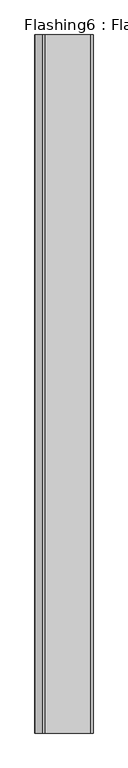
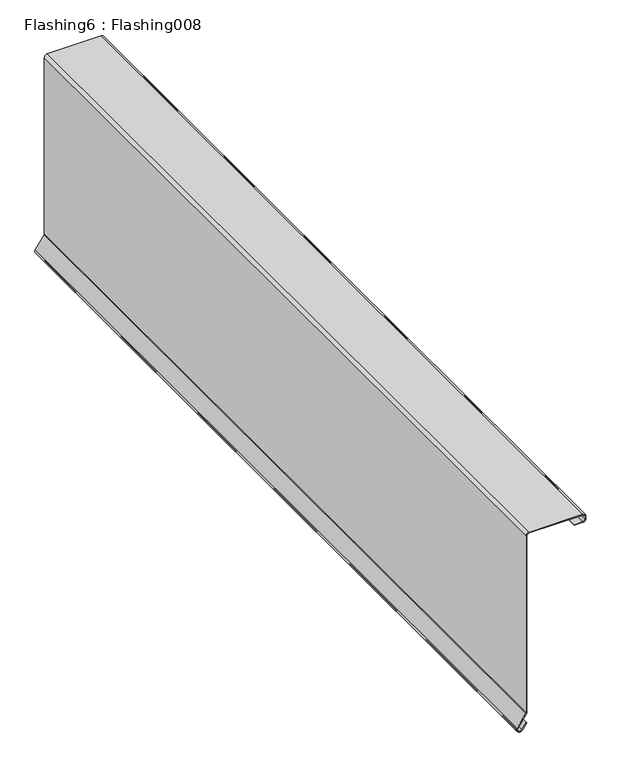
"""IFC4 building model written with IfcOpenShell, lengths in millimetres: proxy geometry, Flashing6 : Flashing008."""

import ifcopenshell
import ifcopenshell.guid

model = None  # the IFC model being written
_history = None  # IfcOwnerHistory: only IFC2X3 demands one
_inside = {}  # id of a spatial element -> (the spatial element, [elements in it])
_under = {}  # id of a project, library or spatial element -> (it, [spatial elements below it])
_declared = {}  # id of a project -> (the project, [libraries it declares])
_typed = {}  # id of a type object -> (the type object, [elements of that type])
_made_of = {}  # id of a material, layer set ... -> (it, [elements and type objects made of it])


def new_model(schema):
    """Start an empty IFC model of exactly this schema.

    Asked for "IFC4X3", IfcOpenShell would pick the latest addendum, in which some entities
    have other attributes; the version numbers below select the first issue.
    IFC2X3 requires an IfcOwnerHistory on every rooted entity: one is made here for all.
    """
    global model, _history
    if schema == "IFC4X3":
        model = ifcopenshell.file(schema_version=(4, 3, 0, 0))
    else:
        model = ifcopenshell.file(schema=schema)
    _inside.clear()
    _under.clear()
    _declared.clear()
    _typed.clear()
    _made_of.clear()
    _history = None
    if model.schema == "IFC2X3":
        org = make("IfcOrganization", Name="unknown")
        user = make(
            "IfcPersonAndOrganization",
            ThePerson=make("IfcPerson", FamilyName="unknown"),
            TheOrganization=org,
        )
        app = make(
            "IfcApplication",
            ApplicationDeveloper=org,
            Version="unknown",
            ApplicationFullName="unknown",
            ApplicationIdentifier="unknown",
        )
        _history = make(
            "IfcOwnerHistory",
            OwningUser=user,
            OwningApplication=app,
            ChangeAction="ADDED",
            CreationDate=0,
        )
    return model


def make(cls, **values):
    """One entity of the class cls with the attributes given. An attribute that is None is left unset."""
    return model.create_entity(
        cls, **{name: value for name, value in values.items() if value is not None}
    )


def rooted(cls, **values):
    """An entity with a GlobalId (a new one), such as an element, a storey or a relation."""
    return make(cls, GlobalId=ifcopenshell.guid.new(), OwnerHistory=_history, **values)


def si_unit(unit_type, name, prefix=None):
    """IfcSIUnit, for example si_unit("LENGTHUNIT", "METRE", prefix="MILLI")."""
    return make("IfcSIUnit", UnitType=unit_type, Prefix=prefix, Name=name)


def assignment(units):
    """IfcUnitAssignment: the units of a project."""
    return None if units is None else make("IfcUnitAssignment", Units=units)


def point(xyz):
    """IfcCartesianPoint."""
    return None if xyz is None else make("IfcCartesianPoint", Coordinates=xyz)


def direction(xyz):
    """IfcDirection."""
    return None if xyz is None else make("IfcDirection", DirectionRatios=xyz)


def frame(location, z_axis=None, x_axis=None):
    """IfcAxis2Placement3D, a coordinate frame: its origin and axes. An axis left out is left unset."""
    return make(
        "IfcAxis2Placement3D",
        Location=point(location),
        Axis=direction(z_axis),
        RefDirection=direction(x_axis),
    )


def frame_2d(location, x_axis=None):
    """IfcAxis2Placement2D, a coordinate frame in the plane: its origin and x axis."""
    return make(
        "IfcAxis2Placement2D", Location=point(location), RefDirection=direction(x_axis)
    )


def origin():
    """The frame at (0, 0, 0) with its axes left unset."""
    return frame((0.0, 0.0, 0.0))


def place(relative_to, where):
    """IfcLocalPlacement: puts the frame where relative to a parent placement (None: the world)."""
    return make(
        "IfcLocalPlacement", PlacementRelTo=relative_to, RelativePlacement=where
    )


def context(
    kind, dimensions, precision=None, world=None, true_north=None, identifier=None
):
    """IfcGeometricRepresentationContext, for example the 3D "Model" context."""
    return make(
        "IfcGeometricRepresentationContext",
        ContextIdentifier=identifier,
        ContextType=kind,
        CoordinateSpaceDimension=dimensions,
        Precision=precision,
        WorldCoordinateSystem=world,
        TrueNorth=true_north,
    )


def project(units=None, contexts=None):
    """IfcProject with its units and contexts."""
    return rooted(
        "IfcProject",
        Name="project",
        RepresentationContexts=contexts,
        UnitsInContext=assignment(units),
    )


def spatial(cls, under=None, at=None, **own):
    """A site, building, storey or space (cls), placed at a placement, below another one or the project."""
    s = rooted(cls, ObjectPlacement=at, **own)
    if under is not None:
        _under.setdefault(under.id(), (under, []))[1].append(s)
    return s


def polyline(points):
    """IfcPolyline through the points."""
    return make("IfcPolyline", Points=[point(p) for p in points])


def circle_curve(where, radius):
    """IfcCircle in the frame where."""
    return make("IfcCircle", Position=where, Radius=radius)


def trimmed(basis, trim1, trim2, sense, master):
    """IfcTrimmedCurve: the piece of a basis curve between two trims."""
    return make(
        "IfcTrimmedCurve",
        BasisCurve=basis,
        Trim1=trim1,
        Trim2=trim2,
        SenseAgreement=sense,
        MasterRepresentation=master,
    )


def segment(curve, same_sense, transition):
    """IfcCompositeCurveSegment."""
    return make(
        "IfcCompositeCurveSegment",
        Transition=transition,
        SameSense=same_sense,
        ParentCurve=curve,
    )


def composite_curve(segments, self_intersect=None):
    """IfcCompositeCurve: segments joined end to end."""
    return make("IfcCompositeCurve", Segments=segments, SelfIntersect=self_intersect)


def outline(outer, holes=None, kind="AREA"):
    """IfcArbitraryClosedProfileDef: a profile drawn as a closed curve; with holes, ...WithVoids."""
    if holes is None:
        return make("IfcArbitraryClosedProfileDef", ProfileType=kind, OuterCurve=outer)
    return make(
        "IfcArbitraryProfileDefWithVoids",
        ProfileType=kind,
        OuterCurve=outer,
        InnerCurves=holes,
    )


def extrude(swept, where, along, depth):
    """IfcExtrudedAreaSolid: the profile swept, set in the frame where, extruded along a direction by depth."""
    return make(
        "IfcExtrudedAreaSolid",
        SweptArea=swept,
        Position=where,
        ExtrudedDirection=direction(along),
        Depth=depth,
    )


def shape(context_of_items, identifier, shape_type, items):
    """IfcShapeRepresentation: the items that make up one representation, for example the "Body"."""
    return make(
        "IfcShapeRepresentation",
        ContextOfItems=context_of_items,
        RepresentationIdentifier=identifier,
        RepresentationType=shape_type,
        Items=items,
    )


def source(mapping_origin, context_of_items, identifier, shape_type, items):
    """IfcRepresentationMap: a shape defined once, which mapped items show again and again."""
    return make(
        "IfcRepresentationMap",
        MappingOrigin=mapping_origin,
        MappedRepresentation=shape(context_of_items, identifier, shape_type, items),
    )


def transform(
    local_origin,
    x_axis=None,
    y_axis=None,
    z_axis=None,
    scale=None,
    scale2=None,
    scale3=None,
    uniform=True,
):
    """IfcCartesianTransformationOperator3D, or its non-uniform kind. x_axis, y_axis, z_axis: its Axis1, 2, 3."""
    if uniform:
        return make(
            "IfcCartesianTransformationOperator3D",
            Axis1=direction(x_axis),
            Axis2=direction(y_axis),
            LocalOrigin=point(local_origin),
            Scale=scale,
            Axis3=direction(z_axis),
        )
    return make(
        "IfcCartesianTransformationOperator3DnonUniform",
        Axis1=direction(x_axis),
        Axis2=direction(y_axis),
        LocalOrigin=point(local_origin),
        Scale=scale,
        Axis3=direction(z_axis),
        Scale2=scale2,
        Scale3=scale3,
    )


def mapped(mapping_source, mapping_target):
    """IfcMappedItem: shows the shape of a source again, moved by a transform."""
    return make(
        "IfcMappedItem", MappingSource=mapping_source, MappingTarget=mapping_target
    )


def made_of(thing, what):
    """Note that an element or type object is made of a material, layer set ...; save() writes the relation."""
    if what is not None:
        _made_of.setdefault(what.id(), (what, []))[1].append(thing)
    return thing


def element(
    cls,
    number,
    at=None,
    inside=None,
    cuts=None,
    type_object=None,
    material=None,
    context=None,
    identifier="Body",
    shape_type=None,
    held_by="IfcProductDefinitionShape",
    body=None,
    shapes=None,
    **own,
):
    """One element of the class cls, such as IfcWall. Its Tag is "e" and its number.

    at: its placement. inside: the storey or other place that contains it. cuts: it is an
    opening in that element (IfcRelVoidsElement). A single representation is given by context,
    identifier, shape_type and body (its items); several are given by shapes. held_by: the class
    of the entity that holds the representations. save() writes the other relations.
    """
    e = rooted(cls, Tag="e%d" % number, ObjectPlacement=at, **own)
    if body is not None:
        shapes = [shape(context, identifier, shape_type, body)]
    if shapes is not None:
        e.Representation = make(held_by, Representations=shapes)
    if inside is not None:
        _inside.setdefault(inside.id(), (inside, []))[1].append(e)
    if cuts is not None:
        rooted(
            "IfcRelVoidsElement", RelatingBuildingElement=cuts, RelatedOpeningElement=e
        )
    if type_object is not None:
        _typed.setdefault(type_object.id(), (type_object, []))[1].append(e)
    return made_of(e, material)


def aggregate(whole, parts):
    """IfcRelAggregates: a whole, such as a stair, and the parts it consists of."""
    return rooted("IfcRelAggregates", RelatingObject=whole, RelatedObjects=parts)


def save(model, path):
    """Write the relations noted so far, then the file.

    IfcRelAggregates (storeys below a building ...), IfcRelContainedInSpatialStructure (elements
    in a storey), IfcRelDefinesByType, IfcRelAssociatesMaterial and IfcRelDeclares: one each for
    every whole, place, type object, material and project.
    """
    for whole, parts in _under.values():
        aggregate(whole, parts)
    for where, things in _inside.values():
        rooted(
            "IfcRelContainedInSpatialStructure",
            RelatedElements=things,
            RelatingStructure=where,
        )
    for kind, things in _typed.values():
        rooted("IfcRelDefinesByType", RelatedObjects=things, RelatingType=kind)
    for what, things in _made_of.values():
        rooted("IfcRelAssociatesMaterial", RelatedObjects=things, RelatingMaterial=what)
    for by, libraries in _declared.values():
        rooted("IfcRelDeclares", RelatingContext=by, RelatedDefinitions=libraries)
    model.write(path)


def flashing6_flashing008_516c5e6e(model_context):
    return source(origin(), model_context, "Body", "SweptSolid", [
        extrude(outline(composite_curve([segment(trimmed(circle_curve(frame_2d((43033.8898747, -6514.9327408)), 5.08), [point((43030.9678143, -6510.7772669))], [point((43029.7783694, -6517.9163501))], True, "CARTESIAN"), True, "CONTINUOUS"), segment(polyline([(43029.7783694, -6517.9163501), (43031.0710485, -6519.6977016)]), True, "CONTINUOUS"), segment(trimmed(circle_curve(frame_2d((43035.1825538, -6516.7140923)), 5.08), [point((43031.0710485, -6519.6977016))], [point((43038.0896432, -6520.8800533))], True, "CARTESIAN"), True, "CONTINUOUS"), segment(polyline([(43038.0896432, -6520.8800533), (43068.3424938, -6499.7690195)]), True, "CONTINUOUS"), segment(trimmed(circle_curve(frame_2d((43071.2495833, -6503.9349805)), 5.08), [point((43068.3424938, -6499.7690195))], [point((43071.2495833, -6498.8549805))], False, "CARTESIAN"), True, "CONTINUOUS"), segment(polyline([(43071.2495833, -6498.8549805), (43518.4785937, -6498.8549805)]), True, "CONTINUOUS"), segment(trimmed(circle_curve(frame_2d((43518.4785937, -6493.7749805)), 5.08), [point((43518.4785937, -6498.8549805))], [point((43523.5585937, -6493.7749805))], True, "CARTESIAN"), True, "CONTINUOUS"), segment(polyline([(43523.5585937, -6493.7749805), (43523.5585937, -6364.4349805)]), True, "CONTINUOUS"), segment(trimmed(circle_curve(frame_2d((43518.4785937, -6364.4349805)), 5.08), [point((43523.5585937, -6364.4349805))], [point((43518.4785937, -6359.3549805))], True, "CARTESIAN"), True, "CONTINUOUS"), segment(polyline([(43518.4785937, -6359.3549805), (43512.0721875, -6359.3549805)]), True, "CONTINUOUS"), segment(trimmed(circle_curve(frame_2d((43512.0721875, -6364.4349805)), 5.08), [point((43512.0721875, -6359.3549805))], [point((43506.9921875, -6364.4349805))], True, "CARTESIAN"), True, "CONTINUOUS"), segment(polyline([(43506.9921875, -6364.4349805), (43506.9921875, -6385.7314453), (43504.9921875, -6385.7314453), (43504.9921875, -6364.4349805)]), True, "CONTINUOUS"), segment(trimmed(circle_curve(frame_2d((43512.0721875, -6364.4349805)), 7.08), [point((43504.9921875, -6364.4349805))], [point((43512.0721875, -6357.3549805))], False, "CARTESIAN"), True, "CONTINUOUS"), segment(polyline([(43512.0721875, -6357.3549805), (43518.4785937, -6357.3549805)]), True, "CONTINUOUS"), segment(trimmed(circle_curve(frame_2d((43518.4785937, -6364.4349805)), 7.08), [point((43518.4785937, -6357.3549805))], [point((43525.5585937, -6364.4349805))], False, "CARTESIAN"), True, "CONTINUOUS"), segment(polyline([(43525.5585937, -6364.4349805), (43525.5585937, -6493.7749805)]), True, "CONTINUOUS"), segment(trimmed(circle_curve(frame_2d((43518.4785937, -6493.7749805)), 7.08), [point((43525.5585937, -6493.7749805))], [point((43518.4785937, -6500.8549805))], False, "CARTESIAN"), True, "CONTINUOUS"), segment(polyline([(43518.4785937, -6500.8549805), (43071.2495833, -6500.8549805)]), True, "CONTINUOUS"), segment(trimmed(circle_curve(frame_2d((43071.2495833, -6503.9349805)), 3.08), [point((43071.2495833, -6500.8549805))], [point((43069.4870172, -6501.4091616))], True, "CARTESIAN"), True, "CONTINUOUS"), segment(polyline([(43069.4870172, -6501.4091616), (43039.2341666, -6522.5201954)]), True, "CONTINUOUS"), segment(trimmed(circle_curve(frame_2d((43035.1825538, -6516.7140923)), 7.08), [point((43039.2341666, -6522.5201954))], [point((43029.4523457, -6520.872351))], False, "CARTESIAN"), True, "CONTINUOUS"), segment(polyline([(43029.4523457, -6520.872351), (43028.1596666, -6519.0909995)]), True, "CONTINUOUS"), segment(trimmed(circle_curve(frame_2d((43033.8898747, -6514.9327408)), 7.08), [point((43028.1596666, -6519.0909995))], [point((43029.8173969, -6509.1412536))], False, "CARTESIAN"), True, "CONTINUOUS"), segment(polyline([(43029.8173969, -6509.1412536), (43044.40427, -6498.8840062), (43045.5546875, -6500.5200195), (43030.9678143, -6510.7772669)]), True, "CONTINUOUS")], self_intersect=False)), frame((0.0, 7982.1531721, 0.0), z_axis=(0.0, 1.0, 0.0), x_axis=(0.0, 0.0, 1.0)), (0.0, 0.0, 1.0), 2000.0),
    ])


if __name__ == "__main__":
    model = new_model("IFC4")
    model_context = context("Model", 3, world=origin())
    ifc_project = project(units=[si_unit("LENGTHUNIT", "METRE", prefix="MILLI")], contexts=[model_context])
    site = spatial("IfcSite", under=ifc_project)
    building = spatial("IfcBuilding", under=site)
    placement = place(None, origin())
    flashing6_flashing008_shape = flashing6_flashing008_516c5e6e(model_context)
    element("IfcBuildingElementProxy", 1, Name="Flashing6 : Flashing008", ObjectType="Flashing6 : Flashing008", at=placement, inside=building, context=model_context, shape_type="MappedRepresentation", body=[
        mapped(flashing6_flashing008_shape, transform((0.0, 0.0, 0.0), x_axis=(1.0, 0.0, 0.0), y_axis=(0.0, 1.0, 0.0), z_axis=(0.0, 0.0, 1.0))),
    ])
    save(model, "model.ifc")

# Revit data of these elements
# Type "Flashing6 : Flashing008"
#   NameOverride = "Flashing008"
# Element 1 (IfcBuildingElementProxy, "Flashing6 : Flashing008")
#   Materials on its faces: "BRAKE METAL EAVE TRIM TO MATCH STANDING SEAM COLOR"
# Materials
#   "BRAKE METAL EAVE TRIM TO MATCH STANDING SEAM COLOR": class "Unassigned", colour RGB 128 128 128, transparency 0, Cost = 0
